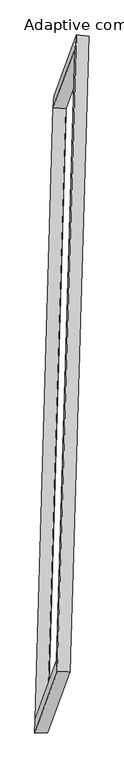
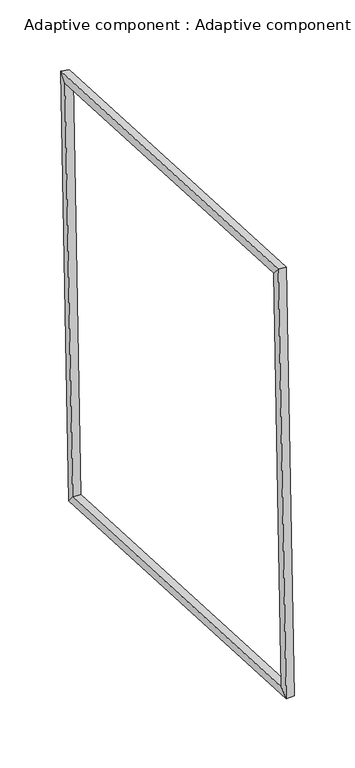
"""IFC4 building model written with IfcOpenShell, lengths in millimetres: proxy geometry, Adaptive component : Adaptive component."""

from ifc_helpers import new_model, si_unit, origin, place, context, project, spatial, faceted_brep, source, transform, mapped, element, save


def adaptive_component_adaptive_component_dea4b03b(model_context):
    return source(origin(), model_context, "Body", "Brep", [
        faceted_brep([(78.6038214, 1289.7612221, 2884.9244707), (143.2369891, 1283.9371665, 2879.9006183), (49.423427, -1827.4612721, 3160.6167775), (-15.4142476, -1828.4198448, 3166.2525713), (86.0765552, 1360.0344995, 2943.6119451), (-11.8382403, -1887.3844782, 3236.6001306), (150.7097229, 1354.2104439, 2938.5880926), (52.9994343, -1886.4259055, 3230.9643368), (-60.5950994, -2126.5414088, -191.0915916), (-125.6554122, -2128.1052128, -192.2384573), (-126.3216087, -2198.6020756, -251.1294026), (-61.2612958, -2197.0382716, -249.9825369), (33.2184626, 984.8570297, -471.8077509), (-31.6373432, 990.0758541, -473.5665579), (-28.4068132, 1048.8169021, -544.1175881), (36.4489927, 1043.5980778, -542.3587811)], [[[0, 1, 2, 3]], [[4, 0, 3, 5]], [[6, 4, 5, 7]], [[1, 6, 7, 2]], [[3, 2, 8, 9]], [[5, 3, 9, 10]], [[7, 5, 10, 11]], [[2, 7, 11, 8]], [[9, 8, 12, 13]], [[10, 9, 13, 14]], [[11, 10, 14, 15]], [[8, 11, 15, 12]], [[13, 12, 1, 0]], [[14, 13, 0, 4]], [[15, 14, 4, 6]], [[12, 15, 6, 1]]]),
    ])


if __name__ == "__main__":
    model = new_model("IFC4")
    model_context = context("Model", 3, world=origin())
    ifc_project = project(units=[si_unit("LENGTHUNIT", "METRE", prefix="MILLI")], contexts=[model_context])
    site = spatial("IfcSite", under=ifc_project)
    building = spatial("IfcBuilding", under=site)
    placement = place(None, origin())
    adaptive_component_adaptive_component_shape = adaptive_component_adaptive_component_dea4b03b(model_context)
    element("IfcBuildingElementProxy", 1, Name="Adaptive component : Adaptive component", ObjectType="Adaptive component : Adaptive component", at=placement, inside=building, context=model_context, shape_type="MappedRepresentation", body=[
        mapped(adaptive_component_adaptive_component_shape, transform((0.0, 0.0, 0.0), x_axis=(1.0, 0.0, 0.0), y_axis=(0.0, 1.0, 0.0), z_axis=(0.0, 0.0, 1.0))),
    ])
    save(model, "model.ifc")

# Revit data of these elements
# Type "Adaptive component : Adaptive component"
#   r [instance default] = 2063.125 mm
#   2r [instance default] = 4126.251 mm
#   Number [instance default] = 5
#   Default Elevation = 0
# Element 1 (IfcBuildingElementProxy, "Adaptive component : Adaptive component")
#   r = 2391.057 mm
#   2r = 4782.113 mm
#   Number = 17
